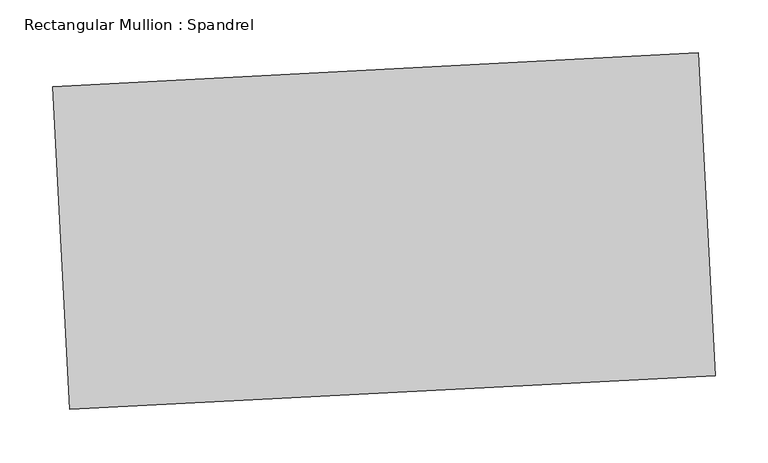
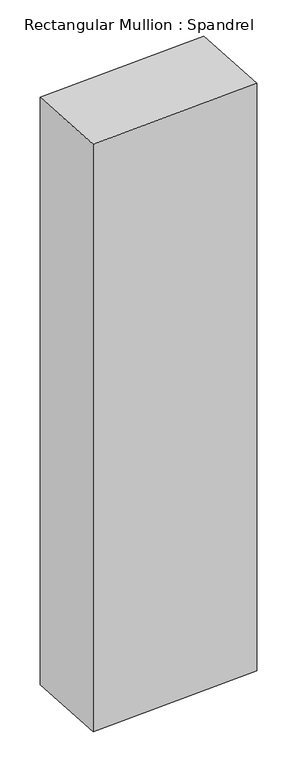
"""IFC4 building model written with IfcOpenShell, lengths in millimetres: member geometry, Rectangular Mullion : Spandrel."""

from ifc_helpers import new_model, si_unit, frame, origin, place, context, project, spatial, polyline, outline, extrude, source, transform, mapped, element, save


def rectangular_mullion_spandrel_39493fd7(model_context):
    return source(origin(), model_context, "Body", "SweptSolid", [
        extrude(outline(polyline([(-617.1582819, 136.2391416), (-8.3937175, 168.1431406), (7.5582819, -136.2391416), (-601.2062825, -168.1431406), (-617.1582819, 136.2391416)])), frame((0.0, 0.0, -2238.2640239), z_axis=(0.0, 0.0, 1.0), x_axis=(1.0, 0.0, 0.0)), (0.0, 0.0, 1.0), 2238.2640239),
    ])


if __name__ == "__main__":
    model = new_model("IFC4")
    model_context = context("Model", 3, world=origin())
    ifc_project = project(units=[si_unit("LENGTHUNIT", "METRE", prefix="MILLI")], contexts=[model_context])
    site = spatial("IfcSite", under=ifc_project)
    building = spatial("IfcBuilding", under=site)
    placement = place(None, origin())
    rectangular_mullion_spandrel_shape = rectangular_mullion_spandrel_39493fd7(model_context)
    element("IfcMember", 1, ObjectType="Rectangular Mullion : Spandrel", at=placement, inside=building, context=model_context, shape_type="MappedRepresentation", body=[
        mapped(rectangular_mullion_spandrel_shape, transform((0.0, 0.0, 0.0), x_axis=(1.0, 0.0, 0.0), y_axis=(0.0, 1.0, 0.0), z_axis=(0.0, 0.0, 1.0))),
    ])
    save(model, "model.ifc")

# Revit data of these elements
# Type "Rectangular Mullion : Spandrel"
#   built-in parameter 1007304 = 1 (stored number, unit not read)
#   built-in parameter 1007301 = 1 (stored number, unit not read)
#   built-in parameter 1007300 = 1 (stored number, unit not read)
# Element 1 (IfcMember, "Rectangular Mullion : Spandrel")
#   Materials on its faces: "Aluminum"
# Materials
#   "Aluminum": class "Metal", colour RGB 247 247 247, transparency 0, Description = "Aluminum 6061", Cost = 0
